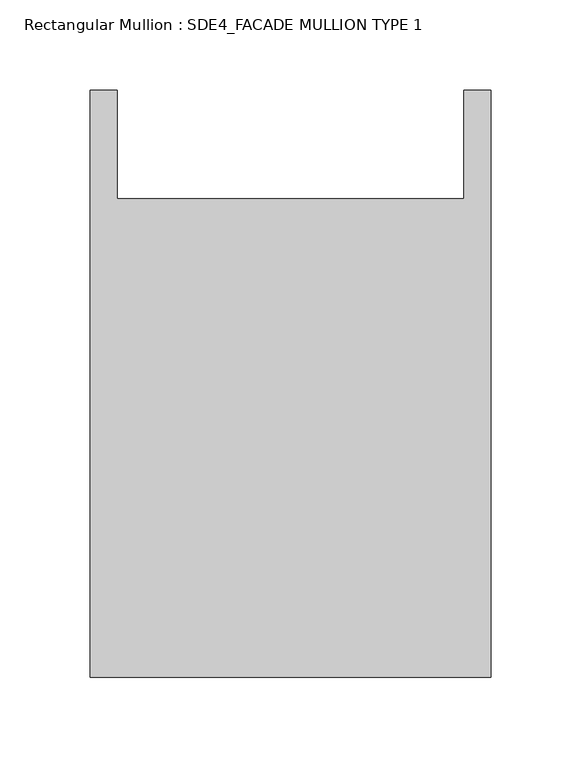
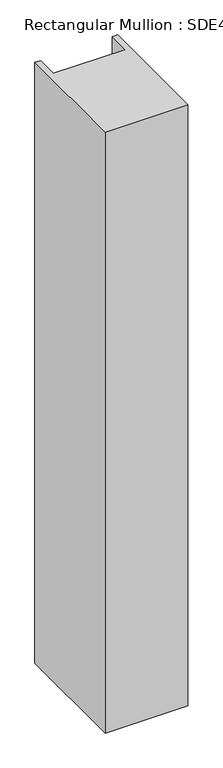
"""IFC4 building model written with IfcOpenShell, lengths in millimetres: member geometry, Rectangular Mullion : SDE4_FACADE MULLION TYPE 1."""

from ifc_helpers import new_model, si_unit, frame, origin, place, context, project, spatial, polyline, outline, extrude, source, transform, mapped, element, save


def rectangular_mullion_sde4_facade_mullion_type_1_fbcf9c1a(model_context):
    return source(origin(), model_context, "Body", "SweptSolid", [
        extrude(outline(polyline([(111.0, -132.5), (-111.0, -132.5), (-111.0, 192.5), (-96.0, 192.5), (-96.0, 132.5), (96.0, 132.5), (96.0, 192.5), (111.0, 192.5), (111.0, -132.5)])), frame((0.0, 0.0, -1700.4043686), z_axis=(0.0, 0.0, 1.0), x_axis=(1.0, 0.0, 0.0)), (0.0, 0.0, 1.0), 1700.4043686),
    ])


if __name__ == "__main__":
    model = new_model("IFC4")
    model_context = context("Model", 3, world=origin())
    ifc_project = project(units=[si_unit("LENGTHUNIT", "METRE", prefix="MILLI")], contexts=[model_context])
    site = spatial("IfcSite", under=ifc_project)
    building = spatial("IfcBuilding", under=site)
    placement = place(None, origin())
    rectangular_mullion_sde4_facade_mullion_type_1_shape = rectangular_mullion_sde4_facade_mullion_type_1_fbcf9c1a(model_context)
    element("IfcMember", 1, ObjectType="Rectangular Mullion : SDE4_FACADE MULLION TYPE 1", at=placement, inside=building, context=model_context, shape_type="MappedRepresentation", body=[
        mapped(rectangular_mullion_sde4_facade_mullion_type_1_shape, transform((0.0, 0.0, 0.0), x_axis=(1.0, 0.0, 0.0), y_axis=(0.0, 1.0, 0.0), z_axis=(0.0, 0.0, 1.0))),
    ])
    save(model, "model.ifc")

# Revit data of these elements
# Type "Rectangular Mullion : SDE4_FACADE MULLION TYPE 1"
#   built-in parameter 1007322 = 0.869423 (stored number, unit not read)
#   built-in parameter 1007321 = 0.364173 (stored number, unit not read)
#   built-in parameter 1007320 = 0.364173 (stored number, unit not read)
